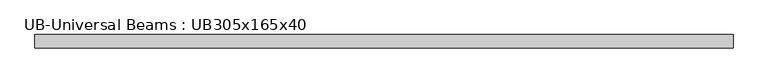
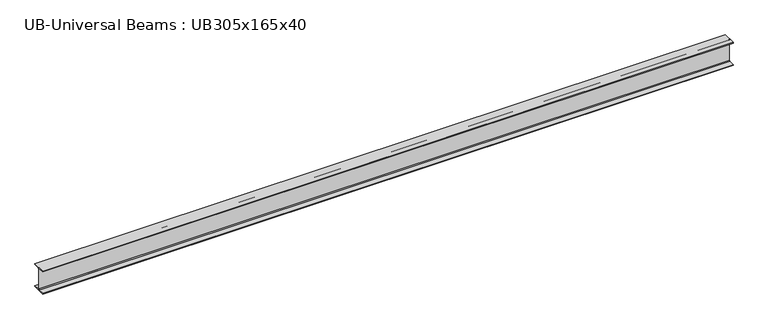
"""IFC4 building model written with IfcOpenShell, lengths in millimetres: beam geometry, UB-Universal Beams : UB305x165x40."""

import ifcopenshell
import ifcopenshell.guid

model = None  # the IFC model being written
_history = None  # IfcOwnerHistory: only IFC2X3 demands one
_inside = {}  # id of a spatial element -> (the spatial element, [elements in it])
_under = {}  # id of a project, library or spatial element -> (it, [spatial elements below it])
_declared = {}  # id of a project -> (the project, [libraries it declares])
_typed = {}  # id of a type object -> (the type object, [elements of that type])
_made_of = {}  # id of a material, layer set ... -> (it, [elements and type objects made of it])


def new_model(schema):
    """Start an empty IFC model of exactly this schema.

    Asked for "IFC4X3", IfcOpenShell would pick the latest addendum, in which some entities
    have other attributes; the version numbers below select the first issue.
    IFC2X3 requires an IfcOwnerHistory on every rooted entity: one is made here for all.
    """
    global model, _history
    if schema == "IFC4X3":
        model = ifcopenshell.file(schema_version=(4, 3, 0, 0))
    else:
        model = ifcopenshell.file(schema=schema)
    _inside.clear()
    _under.clear()
    _declared.clear()
    _typed.clear()
    _made_of.clear()
    _history = None
    if model.schema == "IFC2X3":
        org = make("IfcOrganization", Name="unknown")
        user = make(
            "IfcPersonAndOrganization",
            ThePerson=make("IfcPerson", FamilyName="unknown"),
            TheOrganization=org,
        )
        app = make(
            "IfcApplication",
            ApplicationDeveloper=org,
            Version="unknown",
            ApplicationFullName="unknown",
            ApplicationIdentifier="unknown",
        )
        _history = make(
            "IfcOwnerHistory",
            OwningUser=user,
            OwningApplication=app,
            ChangeAction="ADDED",
            CreationDate=0,
        )
    return model


def make(cls, **values):
    """One entity of the class cls with the attributes given. An attribute that is None is left unset."""
    return model.create_entity(
        cls, **{name: value for name, value in values.items() if value is not None}
    )


def rooted(cls, **values):
    """An entity with a GlobalId (a new one), such as an element, a storey or a relation."""
    return make(cls, GlobalId=ifcopenshell.guid.new(), OwnerHistory=_history, **values)


def si_unit(unit_type, name, prefix=None):
    """IfcSIUnit, for example si_unit("LENGTHUNIT", "METRE", prefix="MILLI")."""
    return make("IfcSIUnit", UnitType=unit_type, Prefix=prefix, Name=name)


def assignment(units):
    """IfcUnitAssignment: the units of a project."""
    return None if units is None else make("IfcUnitAssignment", Units=units)


def point(xyz):
    """IfcCartesianPoint."""
    return None if xyz is None else make("IfcCartesianPoint", Coordinates=xyz)


def direction(xyz):
    """IfcDirection."""
    return None if xyz is None else make("IfcDirection", DirectionRatios=xyz)


def frame(location, z_axis=None, x_axis=None):
    """IfcAxis2Placement3D, a coordinate frame: its origin and axes. An axis left out is left unset."""
    return make(
        "IfcAxis2Placement3D",
        Location=point(location),
        Axis=direction(z_axis),
        RefDirection=direction(x_axis),
    )


def frame_2d(location, x_axis=None):
    """IfcAxis2Placement2D, a coordinate frame in the plane: its origin and x axis."""
    return make(
        "IfcAxis2Placement2D", Location=point(location), RefDirection=direction(x_axis)
    )


def origin():
    """The frame at (0, 0, 0) with its axes left unset."""
    return frame((0.0, 0.0, 0.0))


def place(relative_to, where):
    """IfcLocalPlacement: puts the frame where relative to a parent placement (None: the world)."""
    return make(
        "IfcLocalPlacement", PlacementRelTo=relative_to, RelativePlacement=where
    )


def context(
    kind, dimensions, precision=None, world=None, true_north=None, identifier=None
):
    """IfcGeometricRepresentationContext, for example the 3D "Model" context."""
    return make(
        "IfcGeometricRepresentationContext",
        ContextIdentifier=identifier,
        ContextType=kind,
        CoordinateSpaceDimension=dimensions,
        Precision=precision,
        WorldCoordinateSystem=world,
        TrueNorth=true_north,
    )


def project(units=None, contexts=None):
    """IfcProject with its units and contexts."""
    return rooted(
        "IfcProject",
        Name="project",
        RepresentationContexts=contexts,
        UnitsInContext=assignment(units),
    )


def spatial(cls, under=None, at=None, **own):
    """A site, building, storey or space (cls), placed at a placement, below another one or the project."""
    s = rooted(cls, ObjectPlacement=at, **own)
    if under is not None:
        _under.setdefault(under.id(), (under, []))[1].append(s)
    return s


def polyline(points):
    """IfcPolyline through the points."""
    return make("IfcPolyline", Points=[point(p) for p in points])


def circle_curve(where, radius):
    """IfcCircle in the frame where."""
    return make("IfcCircle", Position=where, Radius=radius)


def trimmed(basis, trim1, trim2, sense, master):
    """IfcTrimmedCurve: the piece of a basis curve between two trims."""
    return make(
        "IfcTrimmedCurve",
        BasisCurve=basis,
        Trim1=trim1,
        Trim2=trim2,
        SenseAgreement=sense,
        MasterRepresentation=master,
    )


def segment(curve, same_sense, transition):
    """IfcCompositeCurveSegment."""
    return make(
        "IfcCompositeCurveSegment",
        Transition=transition,
        SameSense=same_sense,
        ParentCurve=curve,
    )


def composite_curve(segments, self_intersect=None):
    """IfcCompositeCurve: segments joined end to end."""
    return make("IfcCompositeCurve", Segments=segments, SelfIntersect=self_intersect)


def outline(outer, holes=None, kind="AREA"):
    """IfcArbitraryClosedProfileDef: a profile drawn as a closed curve; with holes, ...WithVoids."""
    if holes is None:
        return make("IfcArbitraryClosedProfileDef", ProfileType=kind, OuterCurve=outer)
    return make(
        "IfcArbitraryProfileDefWithVoids",
        ProfileType=kind,
        OuterCurve=outer,
        InnerCurves=holes,
    )


def extrude(swept, where, along, depth):
    """IfcExtrudedAreaSolid: the profile swept, set in the frame where, extruded along a direction by depth."""
    return make(
        "IfcExtrudedAreaSolid",
        SweptArea=swept,
        Position=where,
        ExtrudedDirection=direction(along),
        Depth=depth,
    )


def shape(context_of_items, identifier, shape_type, items):
    """IfcShapeRepresentation: the items that make up one representation, for example the "Body"."""
    return make(
        "IfcShapeRepresentation",
        ContextOfItems=context_of_items,
        RepresentationIdentifier=identifier,
        RepresentationType=shape_type,
        Items=items,
    )


def source(mapping_origin, context_of_items, identifier, shape_type, items):
    """IfcRepresentationMap: a shape defined once, which mapped items show again and again."""
    return make(
        "IfcRepresentationMap",
        MappingOrigin=mapping_origin,
        MappedRepresentation=shape(context_of_items, identifier, shape_type, items),
    )


def transform(
    local_origin,
    x_axis=None,
    y_axis=None,
    z_axis=None,
    scale=None,
    scale2=None,
    scale3=None,
    uniform=True,
):
    """IfcCartesianTransformationOperator3D, or its non-uniform kind. x_axis, y_axis, z_axis: its Axis1, 2, 3."""
    if uniform:
        return make(
            "IfcCartesianTransformationOperator3D",
            Axis1=direction(x_axis),
            Axis2=direction(y_axis),
            LocalOrigin=point(local_origin),
            Scale=scale,
            Axis3=direction(z_axis),
        )
    return make(
        "IfcCartesianTransformationOperator3DnonUniform",
        Axis1=direction(x_axis),
        Axis2=direction(y_axis),
        LocalOrigin=point(local_origin),
        Scale=scale,
        Axis3=direction(z_axis),
        Scale2=scale2,
        Scale3=scale3,
    )


def mapped(mapping_source, mapping_target):
    """IfcMappedItem: shows the shape of a source again, moved by a transform."""
    return make(
        "IfcMappedItem", MappingSource=mapping_source, MappingTarget=mapping_target
    )


def made_of(thing, what):
    """Note that an element or type object is made of a material, layer set ...; save() writes the relation."""
    if what is not None:
        _made_of.setdefault(what.id(), (what, []))[1].append(thing)
    return thing


def element(
    cls,
    number,
    at=None,
    inside=None,
    cuts=None,
    type_object=None,
    material=None,
    context=None,
    identifier="Body",
    shape_type=None,
    held_by="IfcProductDefinitionShape",
    body=None,
    shapes=None,
    **own,
):
    """One element of the class cls, such as IfcWall. Its Tag is "e" and its number.

    at: its placement. inside: the storey or other place that contains it. cuts: it is an
    opening in that element (IfcRelVoidsElement). A single representation is given by context,
    identifier, shape_type and body (its items); several are given by shapes. held_by: the class
    of the entity that holds the representations. save() writes the other relations.
    """
    e = rooted(cls, Tag="e%d" % number, ObjectPlacement=at, **own)
    if body is not None:
        shapes = [shape(context, identifier, shape_type, body)]
    if shapes is not None:
        e.Representation = make(held_by, Representations=shapes)
    if inside is not None:
        _inside.setdefault(inside.id(), (inside, []))[1].append(e)
    if cuts is not None:
        rooted(
            "IfcRelVoidsElement", RelatingBuildingElement=cuts, RelatedOpeningElement=e
        )
    if type_object is not None:
        _typed.setdefault(type_object.id(), (type_object, []))[1].append(e)
    return made_of(e, material)


def aggregate(whole, parts):
    """IfcRelAggregates: a whole, such as a stair, and the parts it consists of."""
    return rooted("IfcRelAggregates", RelatingObject=whole, RelatedObjects=parts)


def save(model, path):
    """Write the relations noted so far, then the file.

    IfcRelAggregates (storeys below a building ...), IfcRelContainedInSpatialStructure (elements
    in a storey), IfcRelDefinesByType, IfcRelAssociatesMaterial and IfcRelDeclares: one each for
    every whole, place, type object, material and project.
    """
    for whole, parts in _under.values():
        aggregate(whole, parts)
    for where, things in _inside.values():
        rooted(
            "IfcRelContainedInSpatialStructure",
            RelatedElements=things,
            RelatingStructure=where,
        )
    for kind, things in _typed.values():
        rooted("IfcRelDefinesByType", RelatedObjects=things, RelatingType=kind)
    for what, things in _made_of.values():
        rooted("IfcRelAssociatesMaterial", RelatedObjects=things, RelatingMaterial=what)
    for by, libraries in _declared.values():
        rooted("IfcRelDeclares", RelatingContext=by, RelatedDefinitions=libraries)
    model.write(path)


def ub_universal_beams_ub305x165x40_6dcc7521(model_context):
    return source(origin(), model_context, "Body", "SweptSolid", [
        extrude(outline(composite_curve([segment(polyline([(82.5, -141.5), (82.5, -151.7), (-82.5, -151.7), (-82.5, -141.5), (-11.9, -141.5)]), True, "CONTINUOUS"), segment(trimmed(circle_curve(frame_2d((-11.9, -132.6)), 8.9), [point((-11.9, -141.5))], [point((-3.0, -132.6))], True, "CARTESIAN"), True, "CONTINUOUS"), segment(polyline([(-3.0, -132.6), (-3.0, 132.6)]), True, "CONTINUOUS"), segment(trimmed(circle_curve(frame_2d((-11.9, 132.6)), 8.9), [point((-3.0, 132.6))], [point((-11.9, 141.5))], True, "CARTESIAN"), True, "CONTINUOUS"), segment(polyline([(-11.9, 141.5), (-82.5, 141.5), (-82.5, 151.7), (82.5, 151.7), (82.5, 141.5), (11.9, 141.5)]), True, "CONTINUOUS"), segment(trimmed(circle_curve(frame_2d((11.9, 132.6)), 8.9), [point((11.9, 141.5))], [point((3.0, 132.6))], True, "CARTESIAN"), True, "CONTINUOUS"), segment(polyline([(3.0, 132.6), (3.0, -132.6)]), True, "CONTINUOUS"), segment(trimmed(circle_curve(frame_2d((11.9, -132.6)), 8.9), [point((3.0, -132.6))], [point((11.9, -141.5))], True, "CARTESIAN"), True, "CONTINUOUS"), segment(polyline([(11.9, -141.5), (82.5, -141.5)]), True, "CONTINUOUS")], self_intersect=False)), frame((-4333.3, 0.0, 0.0), z_axis=(1.0, 0.0, 0.0), x_axis=(0.0, 1.0, 0.0)), (0.0, 0.0, 1.0), 8666.6),
    ])


if __name__ == "__main__":
    model = new_model("IFC4")
    model_context = context("Model", 3, world=origin())
    ifc_project = project(units=[si_unit("LENGTHUNIT", "METRE", prefix="MILLI")], contexts=[model_context])
    site = spatial("IfcSite", under=ifc_project)
    building = spatial("IfcBuilding", under=site)
    placement = place(None, origin())
    ub_universal_beams_ub305x165x40_shape = ub_universal_beams_ub305x165x40_6dcc7521(model_context)
    element("IfcBeam", 1, ObjectType="UB-Universal Beams : UB305x165x40", at=placement, inside=building, context=model_context, shape_type="MappedRepresentation", body=[
        mapped(ub_universal_beams_ub305x165x40_shape, transform((0.0, 0.0, 0.0), x_axis=(1.0, 0.0, 0.0), y_axis=(0.0, 1.0, 0.0), z_axis=(0.0, 0.0, 1.0))),
    ])
    save(model, "model.ifc")

# Revit data of these elements
# Type "UB-Universal Beams : UB305x165x40"
#   Section Name Key = "UB305X165X40"
#   Width = 16.5 cm
#   Web Thickness = 0.6 cm
#   Web Fillet = 0.89 cm
#   Warping Constant = 164000.0 cm⁶
#   Torsional Moment of Inertia = 14.70 cm⁴
#   Section Area = 51.3 cm²
#   Plastic Modulus weak axis = 142.0 cm³
#   Plastic Modulus strong axis = 623.0 cm³
#   Nominal Weight = 40.2999 kgf/m
#   Moment of Inertia weak axis = 764.00 cm⁴
#   Moment of Inertia strong axis = 8503.00 cm⁴
#   Height = 30.34 cm
#   Flange Thickness = 1.02 cm
#   Elastic Modulus weak axis = 92.6 cm³
#   Elastic Modulus strong axis = 560.0 cm³
#   Centroid Vertical = 15.17 cm
#   Centroid Horizontal = 8.25 cm
#   Bolt Spacing = 9.0 cm
#   Length [instance default] = 1500 mm
#   Structural Material [instance default] = Metal - Steel 43-275
#   Type Comments = ""
#   Assembly Code = ""
# Element 1 (IfcBeam, "UB-Universal Beams : UB305x165x40")
#   Materials on its faces: "Metal - Steel 43-275"
# Materials
#   "Metal - Steel 43-275": class "Metal", colour RGB 247 247 247, transparency 0, Cost = 0
